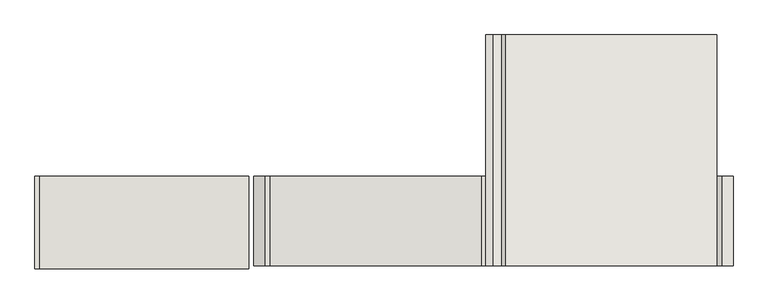
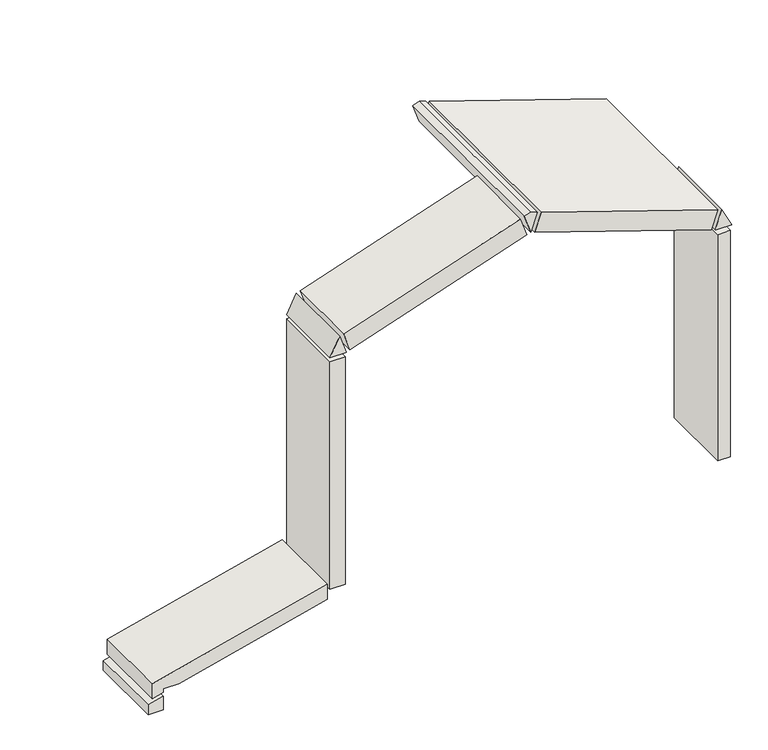
"""IFC4 building model written with IfcOpenShell, lengths in millimetres: wall geometry."""

import ifcopenshell
import ifcopenshell.guid

model = None  # the IFC model being written
_history = None  # IfcOwnerHistory: only IFC2X3 demands one
_inside = {}  # id of a spatial element -> (the spatial element, [elements in it])
_under = {}  # id of a project, library or spatial element -> (it, [spatial elements below it])
_declared = {}  # id of a project -> (the project, [libraries it declares])
_typed = {}  # id of a type object -> (the type object, [elements of that type])
_made_of = {}  # id of a material, layer set ... -> (it, [elements and type objects made of it])


def new_model(schema):
    """Start an empty IFC model of exactly this schema.

    Asked for "IFC4X3", IfcOpenShell would pick the latest addendum, in which some entities
    have other attributes; the version numbers below select the first issue.
    IFC2X3 requires an IfcOwnerHistory on every rooted entity: one is made here for all.
    """
    global model, _history
    if schema == "IFC4X3":
        model = ifcopenshell.file(schema_version=(4, 3, 0, 0))
    else:
        model = ifcopenshell.file(schema=schema)
    _inside.clear()
    _under.clear()
    _declared.clear()
    _typed.clear()
    _made_of.clear()
    _history = None
    if model.schema == "IFC2X3":
        org = make("IfcOrganization", Name="unknown")
        user = make(
            "IfcPersonAndOrganization",
            ThePerson=make("IfcPerson", FamilyName="unknown"),
            TheOrganization=org,
        )
        app = make(
            "IfcApplication",
            ApplicationDeveloper=org,
            Version="unknown",
            ApplicationFullName="unknown",
            ApplicationIdentifier="unknown",
        )
        _history = make(
            "IfcOwnerHistory",
            OwningUser=user,
            OwningApplication=app,
            ChangeAction="ADDED",
            CreationDate=0,
        )
    return model


def make(cls, **values):
    """One entity of the class cls with the attributes given. An attribute that is None is left unset."""
    return model.create_entity(
        cls, **{name: value for name, value in values.items() if value is not None}
    )


def rooted(cls, **values):
    """An entity with a GlobalId (a new one), such as an element, a storey or a relation."""
    return make(cls, GlobalId=ifcopenshell.guid.new(), OwnerHistory=_history, **values)


def si_unit(unit_type, name, prefix=None):
    """IfcSIUnit, for example si_unit("LENGTHUNIT", "METRE", prefix="MILLI")."""
    return make("IfcSIUnit", UnitType=unit_type, Prefix=prefix, Name=name)


def assignment(units):
    """IfcUnitAssignment: the units of a project."""
    return None if units is None else make("IfcUnitAssignment", Units=units)


def point(xyz):
    """IfcCartesianPoint."""
    return None if xyz is None else make("IfcCartesianPoint", Coordinates=xyz)


def direction(xyz):
    """IfcDirection."""
    return None if xyz is None else make("IfcDirection", DirectionRatios=xyz)


def frame(location, z_axis=None, x_axis=None):
    """IfcAxis2Placement3D, a coordinate frame: its origin and axes. An axis left out is left unset."""
    return make(
        "IfcAxis2Placement3D",
        Location=point(location),
        Axis=direction(z_axis),
        RefDirection=direction(x_axis),
    )


def origin():
    """The frame at (0, 0, 0) with its axes left unset."""
    return frame((0.0, 0.0, 0.0))


def place(relative_to, where):
    """IfcLocalPlacement: puts the frame where relative to a parent placement (None: the world)."""
    return make(
        "IfcLocalPlacement", PlacementRelTo=relative_to, RelativePlacement=where
    )


def context(
    kind, dimensions, precision=None, world=None, true_north=None, identifier=None
):
    """IfcGeometricRepresentationContext, for example the 3D "Model" context."""
    return make(
        "IfcGeometricRepresentationContext",
        ContextIdentifier=identifier,
        ContextType=kind,
        CoordinateSpaceDimension=dimensions,
        Precision=precision,
        WorldCoordinateSystem=world,
        TrueNorth=true_north,
    )


def project(units=None, contexts=None):
    """IfcProject with its units and contexts."""
    return rooted(
        "IfcProject",
        Name="project",
        RepresentationContexts=contexts,
        UnitsInContext=assignment(units),
    )


def spatial(cls, under=None, at=None, **own):
    """A site, building, storey or space (cls), placed at a placement, below another one or the project."""
    s = rooted(cls, ObjectPlacement=at, **own)
    if under is not None:
        _under.setdefault(under.id(), (under, []))[1].append(s)
    return s


def polyline(points):
    """IfcPolyline through the points."""
    return make("IfcPolyline", Points=[point(p) for p in points])


def outline(outer, holes=None, kind="AREA"):
    """IfcArbitraryClosedProfileDef: a profile drawn as a closed curve; with holes, ...WithVoids."""
    if holes is None:
        return make("IfcArbitraryClosedProfileDef", ProfileType=kind, OuterCurve=outer)
    return make(
        "IfcArbitraryProfileDefWithVoids",
        ProfileType=kind,
        OuterCurve=outer,
        InnerCurves=holes,
    )


def extrude(swept, where, along, depth):
    """IfcExtrudedAreaSolid: the profile swept, set in the frame where, extruded along a direction by depth."""
    return make(
        "IfcExtrudedAreaSolid",
        SweptArea=swept,
        Position=where,
        ExtrudedDirection=direction(along),
        Depth=depth,
    )


def shape(context_of_items, identifier, shape_type, items):
    """IfcShapeRepresentation: the items that make up one representation, for example the "Body"."""
    return make(
        "IfcShapeRepresentation",
        ContextOfItems=context_of_items,
        RepresentationIdentifier=identifier,
        RepresentationType=shape_type,
        Items=items,
    )


def source(mapping_origin, context_of_items, identifier, shape_type, items):
    """IfcRepresentationMap: a shape defined once, which mapped items show again and again."""
    return make(
        "IfcRepresentationMap",
        MappingOrigin=mapping_origin,
        MappedRepresentation=shape(context_of_items, identifier, shape_type, items),
    )


def transform(
    local_origin,
    x_axis=None,
    y_axis=None,
    z_axis=None,
    scale=None,
    scale2=None,
    scale3=None,
    uniform=True,
):
    """IfcCartesianTransformationOperator3D, or its non-uniform kind. x_axis, y_axis, z_axis: its Axis1, 2, 3."""
    if uniform:
        return make(
            "IfcCartesianTransformationOperator3D",
            Axis1=direction(x_axis),
            Axis2=direction(y_axis),
            LocalOrigin=point(local_origin),
            Scale=scale,
            Axis3=direction(z_axis),
        )
    return make(
        "IfcCartesianTransformationOperator3DnonUniform",
        Axis1=direction(x_axis),
        Axis2=direction(y_axis),
        LocalOrigin=point(local_origin),
        Scale=scale,
        Axis3=direction(z_axis),
        Scale2=scale2,
        Scale3=scale3,
    )


def mapped(mapping_source, mapping_target):
    """IfcMappedItem: shows the shape of a source again, moved by a transform."""
    return make(
        "IfcMappedItem", MappingSource=mapping_source, MappingTarget=mapping_target
    )


def made_of(thing, what):
    """Note that an element or type object is made of a material, layer set ...; save() writes the relation."""
    if what is not None:
        _made_of.setdefault(what.id(), (what, []))[1].append(thing)
    return thing


def element(
    cls,
    number,
    at=None,
    inside=None,
    cuts=None,
    type_object=None,
    material=None,
    context=None,
    identifier="Body",
    shape_type=None,
    held_by="IfcProductDefinitionShape",
    body=None,
    shapes=None,
    **own,
):
    """One element of the class cls, such as IfcWall. Its Tag is "e" and its number.

    at: its placement. inside: the storey or other place that contains it. cuts: it is an
    opening in that element (IfcRelVoidsElement). A single representation is given by context,
    identifier, shape_type and body (its items); several are given by shapes. held_by: the class
    of the entity that holds the representations. save() writes the other relations.
    """
    e = rooted(cls, Tag="e%d" % number, ObjectPlacement=at, **own)
    if body is not None:
        shapes = [shape(context, identifier, shape_type, body)]
    if shapes is not None:
        e.Representation = make(held_by, Representations=shapes)
    if inside is not None:
        _inside.setdefault(inside.id(), (inside, []))[1].append(e)
    if cuts is not None:
        rooted(
            "IfcRelVoidsElement", RelatingBuildingElement=cuts, RelatedOpeningElement=e
        )
    if type_object is not None:
        _typed.setdefault(type_object.id(), (type_object, []))[1].append(e)
    return made_of(e, material)


def aggregate(whole, parts):
    """IfcRelAggregates: a whole, such as a stair, and the parts it consists of."""
    return rooted("IfcRelAggregates", RelatingObject=whole, RelatedObjects=parts)


def save(model, path):
    """Write the relations noted so far, then the file.

    IfcRelAggregates (storeys below a building ...), IfcRelContainedInSpatialStructure (elements
    in a storey), IfcRelDefinesByType, IfcRelAssociatesMaterial and IfcRelDeclares: one each for
    every whole, place, type object, material and project.
    """
    for whole, parts in _under.values():
        aggregate(whole, parts)
    for where, things in _inside.values():
        rooted(
            "IfcRelContainedInSpatialStructure",
            RelatedElements=things,
            RelatingStructure=where,
        )
    for kind, things in _typed.values():
        rooted("IfcRelDefinesByType", RelatedObjects=things, RelatingType=kind)
    for what, things in _made_of.values():
        rooted("IfcRelAssociatesMaterial", RelatedObjects=things, RelatingMaterial=what)
    for by, libraries in _declared.values():
        rooted("IfcRelDeclares", RelatingContext=by, RelatedDefinitions=libraries)
    model.write(path)


def wall_99b056b0(model_context):
    return source(origin(), model_context, "Body", "SweptSolid", [
        extrude(outline(polyline([(5084.8528105, 19749.2870052), (5087.2952862, 19756.5825083), (5261.9187521, 19698.119976), (5084.8528105, 19609.5870052), (5084.8528105, 19749.2870052)])), frame((0.0, -2319.6634634, 0.0), z_axis=(0.0, 1.0, 0.0), x_axis=(0.0, 0.0, 1.0)), (0.0, 0.0, 1.0), 685.8),
        extrude(outline(polyline([(0.0, -1704.0512917), (0.0, 0.0), (685.8, 0.0), (685.8, -1704.0512917), (0.0, -1704.0512917)])), frame((19792.7115012, -2319.6634634, 5099.3909826), z_axis=(-0.3174723447032924, 0.0, 0.9482675309998724), x_axis=(0.0, 1.0, 0.0)), (0.0, 0.0, 1.0), 184.15),
        extrude(outline(polyline([(5652.475838, 21444.7370052), (5827.0993038, 21503.1995375), (5846.6720895, 21444.7370052), (5827.0993038, 21386.2744729), (5652.475838, 21444.7370052)])), frame((0.0, -2319.6634634, 0.0), z_axis=(0.0, 1.0, 0.0), x_axis=(0.0, 0.0, 1.0)), (0.0, 0.0, 1.0), 1767.3456389),
        extrude(outline(polyline([(5084.8528105, 23140.1870052), (5084.8528105, 23279.8870052), (5261.9187521, 23191.3540344), (5087.2952862, 23132.8915021), (5084.8528105, 23140.1870052)])), frame((0.0, -2319.6634634, 0.0), z_axis=(0.0, 1.0, 0.0), x_axis=(0.0, 0.0, 1.0)), (0.0, 0.0, 1.0), 685.8),
        extrude(outline(polyline([(0.0, -1704.0512917), (0.0, 0.0), (1767.345639, 0.0), (1767.345639, -1704.0512917), (0.0, -1704.0512917)])), frame((21480.8659981, -2319.6634634, 5640.3801416), z_axis=(0.3174723447032924, 0.0, 0.9482675309998724), x_axis=(0.0, 1.0, 0.0)), (0.0, 0.0, 1.0), 184.15),
        extrude(outline(polyline([(23267.1870052, -2319.6634634), (23152.8870052, -2319.6634634), (23152.8870052, -1633.8634634), (23267.1870052, -1633.8634634), (23267.1870052, -2319.6634634)])), frame((0.0, 0.0, 2847.975), z_axis=(0.0, 0.0, 1.0), x_axis=(1.0, 0.0, 0.0)), (0.0, 0.0, 1.0), 2186.0778105),
        extrude(outline(polyline([(2922.124464, 19571.4870052), (2522.0767538, 17971.2961644), (2378.0799446, 17971.2961644), (2403.4847319, 18072.8870052), (2438.4, 18072.8870052), (2438.4, 18212.5870052), (2778.125, 19571.4870052), (2922.124464, 19571.4870052)])), frame((0.0, -2344.3317454, 0.0), z_axis=(0.0, 1.0, 0.0), x_axis=(0.0, 0.0, 1.0)), (0.0, 0.0, 1.0), 710.468282),
        extrude(outline(polyline([(2364.2020657, 18072.8870052), (2329.2673338, 17933.1870052), (2235.2, 17933.1870052), (2235.2, 18072.8870052), (2364.2020657, 18072.8870052)])), frame((0.0, -2342.6926084, 0.0), z_axis=(0.0, 1.0, 0.0), x_axis=(0.0, 0.0, 1.0)), (0.0, 0.0, 1.0), 708.8291451),
        extrude(outline(polyline([(19749.2870052, -2319.6634634), (19609.5870052, -2319.6634634), (19609.5870052, -1633.8634634), (19749.2870052, -1633.8634634), (19749.2870052, -2319.6634634)])), frame((0.0, 0.0, 2847.975), z_axis=(0.0, 0.0, 1.0), x_axis=(1.0, 0.0, 0.0)), (0.0, 0.0, 1.0), 2198.7778105),
    ])


if __name__ == "__main__":
    model = new_model("IFC4")
    model_context = context("Model", 3, world=origin())
    ifc_project = project(units=[si_unit("LENGTHUNIT", "METRE", prefix="MILLI")], contexts=[model_context])
    site = spatial("IfcSite", under=ifc_project)
    building = spatial("IfcBuilding", under=site)
    placement = place(None, origin())
    wall_shape = wall_99b056b0(model_context)
    element("IfcWall", 1, ObjectType="2X6'S 16\" O.C. - W/ BATT. INSULATION - VAPOR BARRIER TOWARD INTERIOR : 2X6'S 16\" O.C. - W/ BATT. INSULATION - VAPOR BARRIER TOWARD INTERIOR", at=placement, inside=building, context=model_context, shape_type="MappedRepresentation", body=[
        mapped(wall_shape, transform((0.0, 0.0, 0.0), x_axis=(1.0, 0.0, 0.0), y_axis=(0.0, 1.0, 0.0), z_axis=(0.0, 0.0, 1.0))),
    ])
    save(model, "model.ifc")

# Revit data of these elements
# Element 1 (IfcWall, "2X6'S 16\" O.C. - W/ BATT. INSULATION - VAPOR BARRIER TOWARD INTERIOR : 2X6'S 16\" O.C. - W/ BATT. INSULATION - VAPOR BARRIER TOWARD INTERIOR")
#   Materials on its faces: "POLYURATHANE FOAM (R-43) BETWEEN FIELD FRAMED ROOF (2X8'S)", "2X6 WOOD STUDS @ 16\" O.C. W/ R21 BATT. INSULATION (VAPOR BARRIER TOWARD INTERIOR)", "POLYURATHANE FOAM (R-33) BETWEEN FIELD FRAMED ROOF (2X6'S)"
# Materials
#   "POLYURATHANE FOAM (R-43) BETWEEN FIELD FRAMED ROOF (2X8'S)": class "Unassigned", colour RGB 255 255 255, transparency 0, Cost = 0
#   "2X6 WOOD STUDS @ 16\" O.C. W/ R21 BATT. INSULATION (VAPOR BARRIER TOWARD INTERIOR)": class "Unassigned", colour RGB 255 255 255, transparency 0, Cost = 0
#   "POLYURATHANE FOAM (R-33) BETWEEN FIELD FRAMED ROOF (2X6'S)": class "Unassigned", colour RGB 255 255 255, transparency 0, Cost = 0
